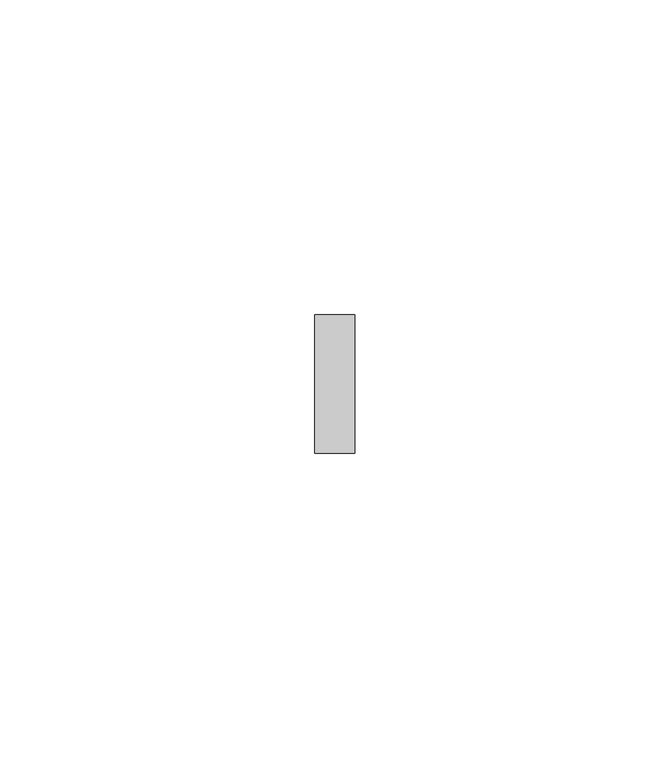
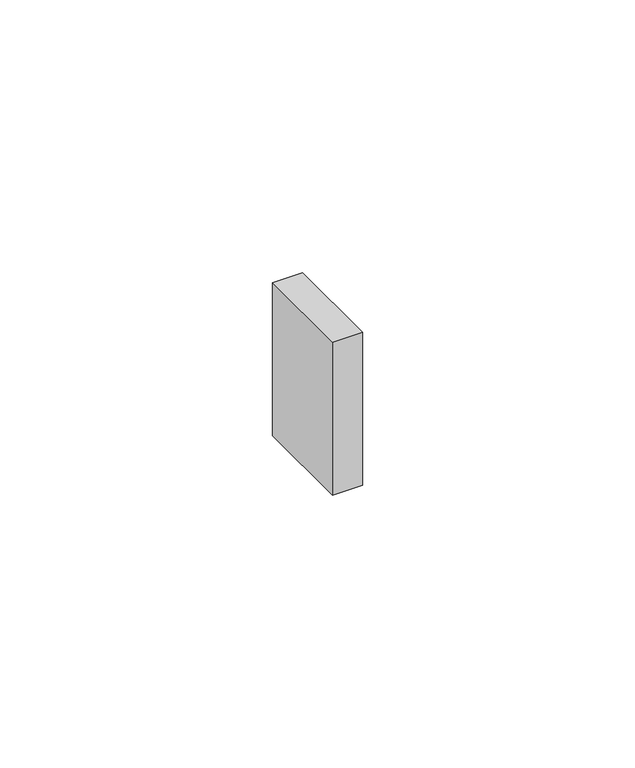
"""IFC4 building model written with IfcOpenShell, lengths in millimetres: proxy geometry, Panel:Panel:300402:Panel:300402 : Panel:Panel:300402:300124:Panel:300402:Panel:300402 : Panel:Panel:300402:300124 : Panel:Panel:300402:Panel:300402 : Panel:Panel:300402:300124:18 : Panel:Panel:300402:Panel:300402 : Panel:Panel:300402:300124:Panel:300402:Panel:300402 : Panel:Panel:300402:300124 : Panel:Panel:300402:Panel:300402 : Panel:Panel:300402:300124:300083."""

from ifc_helpers import new_model, si_unit, frame, origin, place, context, project, spatial, polyline, outline, extrude, source, transform, mapped, element, save


def generic_models_6d84c123(model_context):
    return source(origin(), model_context, "Body", "SweptSolid", [
        extrude(outline(polyline([(560365.6617239, -578686.6186175), (560365.6617239, -578708.5652801), (560359.3117239, -578708.5652801), (560359.3117239, -578686.6186175), (560365.6617239, -578686.6186175)])), frame((0.0, 0.0, 6074.8790379), z_axis=(0.0, 0.0, 1.0), x_axis=(1.0, 0.0, 0.0)), (0.0, 0.0, 1.0), 34.2792892),
    ])


if __name__ == "__main__":
    model = new_model("IFC4")
    model_context = context("Model", 3, world=origin())
    ifc_project = project(units=[si_unit("LENGTHUNIT", "METRE", prefix="MILLI")], contexts=[model_context])
    site = spatial("IfcSite", under=ifc_project)
    building = spatial("IfcBuilding", under=site)
    placement = place(None, origin())
    generic_models_shape = generic_models_6d84c123(model_context)
    element("IfcBuildingElementProxy", 1, Name="Panel:Panel:300402:Panel:300402 : Panel:Panel:300402:300124:Panel:300402:Panel:300402 : Panel:Panel:300402:300124 : Panel:Panel:300402:Panel:300402 : Panel:Panel:300402:300124:18 : Panel:Panel:300402:Panel:300402 : Panel:Panel:300402:300124:Panel:300402:Panel:300402 : Panel:Panel:300402:300124 : Panel:Panel:300402:Panel:300402 : Panel:Panel:300402:300124:300083", ObjectType="Panel:Panel:300402:Panel:300402 : Panel:Panel:300402:300124:Panel:300402:Panel:300402 : Panel:Panel:300402:300124 : Panel:Panel:300402:Panel:300402 : Panel:Panel:300402:300124:18 : Panel:Panel:300402:Panel:300402 : Panel:Panel:300402:300124:Panel:300402:Panel:300402 : Panel:Panel:300402:300124 : Panel:Panel:300402:Panel:300402 : Panel:Panel:300402:300124:300083", at=placement, inside=building, context=model_context, shape_type="MappedRepresentation", body=[
        mapped(generic_models_shape, transform((0.0, 0.0, 0.0), x_axis=(1.0, 0.0, 0.0), y_axis=(0.0, 1.0, 0.0), z_axis=(0.0, 0.0, 1.0))),
    ])
    save(model, "model.ifc")

# Revit data of these elements
# Type "Panel:Panel:300402:Panel:300402 : Panel:Panel:300402:300124:Panel:300402:Panel:300402 : Panel:Panel:300402:300124 : Panel:Panel:300402:Panel:300402 : Panel:Panel:300402:300124:18 : Panel:Panel:300402:Panel:300402 : Panel:Panel:300402:300124:Panel:300402:Panel:300402 : Panel:Panel:300402:300124 : Panel:Panel:300402:Panel:300402 : Panel:Panel:300402:300124:300083"
#   NameOverride = "Panel:Panel:300402:Panel:300402 : Panel:Panel:300402:300124:Panel:300402:Panel:300402 : Panel:Panel:300402:300124 : Panel:Panel:300402:Panel:300402 : Panel:Panel:300402:300124:300083"
#   ObjectTypeOverride = "Panel:300402:Panel:300402 : Panel:Panel:300402:300124 : Panel:Panel:300402:Panel:300402 : Panel:Panel:300402:300124"
#   Reference = "Panel"
#   Tag = "300083"
# Element 1 (IfcBuildingElementProxy, "Panel:Panel:300402:Panel:300402 : Panel:Panel:300402:300124:Panel:300402:Panel:300402 : Panel:Panel:300402:300124 : Panel:Panel:300402:Panel:300402 : Panel:Panel:300402:300124:18 : Panel:Panel:300402:Panel:300402 : Panel:Panel:300402:300124:Panel:300402:Panel:300402 : Panel:Panel:300402:300124 : Panel:Panel:300402:Panel:300402 : Panel:Panel:300402:300124:300083")
#   Materials on its faces: "1/4\" UV & WEATHER RESISTANT SPACER - FROM/BACK OF GIRT"
# Materials
#   "1/4\" UV & WEATHER RESISTANT SPACER - FROM/BACK OF GIRT": class "Unassigned", colour RGB 187 187 187, transparency 0, Keynote = "M07420000.01", Cost = 0
